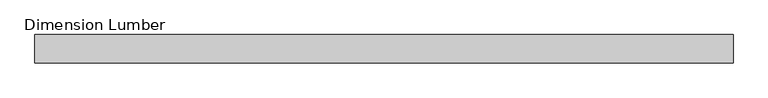
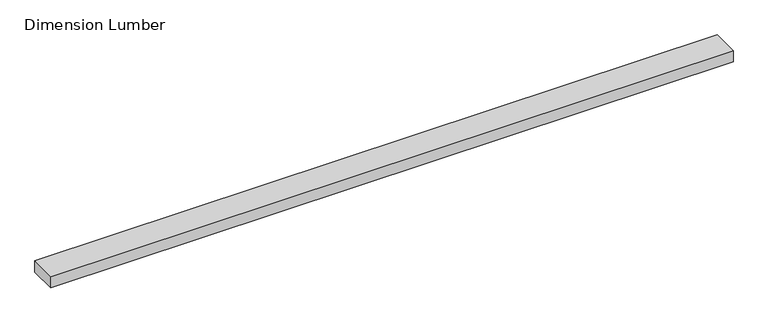
"""IFC4 building model written with IfcOpenShell, lengths in millimetres: beam geometry, Dimension Lumber : Top Supporting Lumbers."""

from ifc_helpers import new_model, si_unit, frame, origin, place, context, project, spatial, polyline, outline, extrude, source, transform, mapped, element, save


def dimension_lumber_2cac8895(model_context):
    return source(origin(), model_context, "Body", "SweptSolid", [
        extrude(outline(polyline([(1119.2453323, 44.45), (1119.2453323, -44.45), (-1074.7953323, -44.45), (-1074.7953323, 44.45), (1119.2453323, 44.45)])), frame((0.0, 0.0, -19.05), z_axis=(0.0, 0.0, 1.0), x_axis=(1.0, 0.0, 0.0)), (0.0, 0.0, 1.0), 38.1),
    ])


if __name__ == "__main__":
    model = new_model("IFC4")
    model_context = context("Model", 3, world=origin())
    ifc_project = project(units=[si_unit("LENGTHUNIT", "METRE", prefix="MILLI")], contexts=[model_context])
    site = spatial("IfcSite", under=ifc_project)
    building = spatial("IfcBuilding", under=site)
    placement = place(None, origin())
    dimension_lumber_shape = dimension_lumber_2cac8895(model_context)
    element("IfcBeam", 1, ObjectType="Dimension Lumber : Top Supporting Lumbers", at=placement, inside=building, context=model_context, shape_type="MappedRepresentation", body=[
        mapped(dimension_lumber_shape, transform((0.0, 0.0, 0.0), x_axis=(1.0, 0.0, 0.0), y_axis=(0.0, 1.0, 0.0), z_axis=(0.0, 0.0, 1.0))),
    ])
    save(model, "model.ifc")

# Revit data of these elements
# Type "Dimension Lumber : Top Supporting Lumbers"
#   Assembly Code = "B10"
#   A = 0.0364583 SF
#   Length [instance default] = 5' - 0"
#   b = 0' - 3 1/2"
#   d = 0' - 1 1/2"
#   Structural Material [instance default] = Softwood, Lumber
# Element 1 (IfcBeam, "Dimension Lumber : Top Supporting Lumbers")
#   Structural Material = Douglas Fir #2
#   Materials on its faces: "Douglas Fir #2"
# Materials
#   "Softwood, Lumber": class "Wood", colour RGB 223 192 134, transparency 0, Description = "Pinus Echinata", Cost = 0
#   "Douglas Fir #2": class "Wood", colour RGB 223 192 134, transparency 0, Description = "Pinus Echinata", Cost = 0
